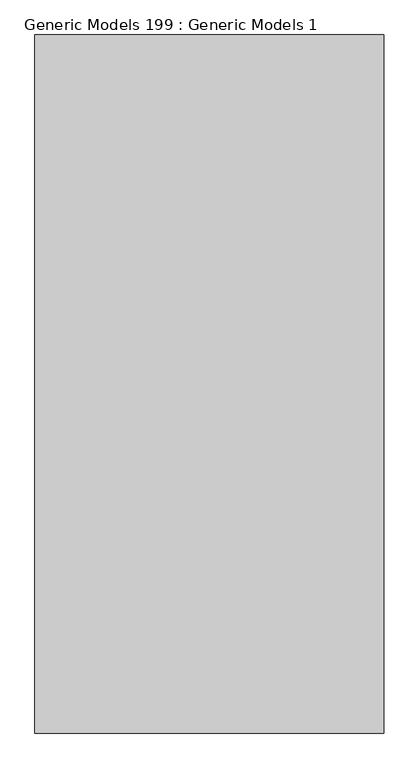
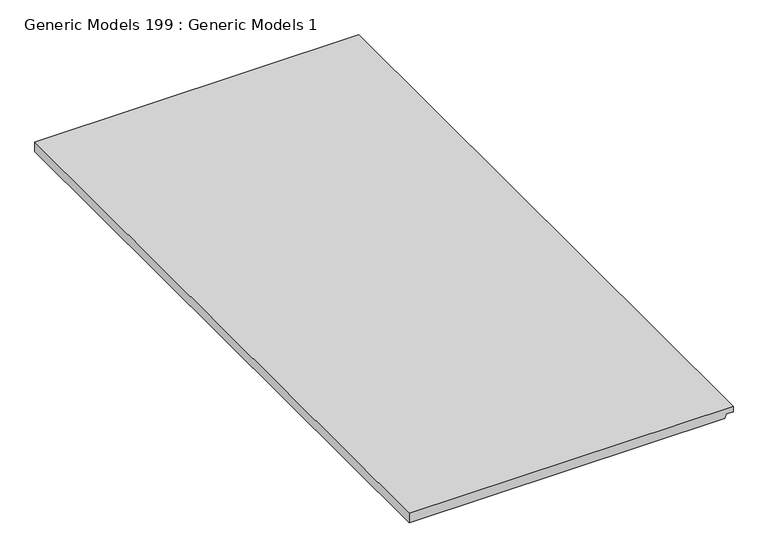
"""IFC4 building model written with IfcOpenShell, lengths in millimetres: proxy geometry, Generic Models 199 : Generic Models 1."""

import ifcopenshell
import ifcopenshell.guid

model = None  # the IFC model being written
_history = None  # IfcOwnerHistory: only IFC2X3 demands one
_inside = {}  # id of a spatial element -> (the spatial element, [elements in it])
_under = {}  # id of a project, library or spatial element -> (it, [spatial elements below it])
_declared = {}  # id of a project -> (the project, [libraries it declares])
_typed = {}  # id of a type object -> (the type object, [elements of that type])
_made_of = {}  # id of a material, layer set ... -> (it, [elements and type objects made of it])


def new_model(schema):
    """Start an empty IFC model of exactly this schema.

    Asked for "IFC4X3", IfcOpenShell would pick the latest addendum, in which some entities
    have other attributes; the version numbers below select the first issue.
    IFC2X3 requires an IfcOwnerHistory on every rooted entity: one is made here for all.
    """
    global model, _history
    if schema == "IFC4X3":
        model = ifcopenshell.file(schema_version=(4, 3, 0, 0))
    else:
        model = ifcopenshell.file(schema=schema)
    _inside.clear()
    _under.clear()
    _declared.clear()
    _typed.clear()
    _made_of.clear()
    _history = None
    if model.schema == "IFC2X3":
        org = make("IfcOrganization", Name="unknown")
        user = make(
            "IfcPersonAndOrganization",
            ThePerson=make("IfcPerson", FamilyName="unknown"),
            TheOrganization=org,
        )
        app = make(
            "IfcApplication",
            ApplicationDeveloper=org,
            Version="unknown",
            ApplicationFullName="unknown",
            ApplicationIdentifier="unknown",
        )
        _history = make(
            "IfcOwnerHistory",
            OwningUser=user,
            OwningApplication=app,
            ChangeAction="ADDED",
            CreationDate=0,
        )
    return model


def make(cls, **values):
    """One entity of the class cls with the attributes given. An attribute that is None is left unset."""
    return model.create_entity(
        cls, **{name: value for name, value in values.items() if value is not None}
    )


def rooted(cls, **values):
    """An entity with a GlobalId (a new one), such as an element, a storey or a relation."""
    return make(cls, GlobalId=ifcopenshell.guid.new(), OwnerHistory=_history, **values)


def si_unit(unit_type, name, prefix=None):
    """IfcSIUnit, for example si_unit("LENGTHUNIT", "METRE", prefix="MILLI")."""
    return make("IfcSIUnit", UnitType=unit_type, Prefix=prefix, Name=name)


def assignment(units):
    """IfcUnitAssignment: the units of a project."""
    return None if units is None else make("IfcUnitAssignment", Units=units)


def point(xyz):
    """IfcCartesianPoint."""
    return None if xyz is None else make("IfcCartesianPoint", Coordinates=xyz)


def direction(xyz):
    """IfcDirection."""
    return None if xyz is None else make("IfcDirection", DirectionRatios=xyz)


def frame(location, z_axis=None, x_axis=None):
    """IfcAxis2Placement3D, a coordinate frame: its origin and axes. An axis left out is left unset."""
    return make(
        "IfcAxis2Placement3D",
        Location=point(location),
        Axis=direction(z_axis),
        RefDirection=direction(x_axis),
    )


def origin():
    """The frame at (0, 0, 0) with its axes left unset."""
    return frame((0.0, 0.0, 0.0))


def place(relative_to, where):
    """IfcLocalPlacement: puts the frame where relative to a parent placement (None: the world)."""
    return make(
        "IfcLocalPlacement", PlacementRelTo=relative_to, RelativePlacement=where
    )


def context(
    kind, dimensions, precision=None, world=None, true_north=None, identifier=None
):
    """IfcGeometricRepresentationContext, for example the 3D "Model" context."""
    return make(
        "IfcGeometricRepresentationContext",
        ContextIdentifier=identifier,
        ContextType=kind,
        CoordinateSpaceDimension=dimensions,
        Precision=precision,
        WorldCoordinateSystem=world,
        TrueNorth=true_north,
    )


def project(units=None, contexts=None):
    """IfcProject with its units and contexts."""
    return rooted(
        "IfcProject",
        Name="project",
        RepresentationContexts=contexts,
        UnitsInContext=assignment(units),
    )


def spatial(cls, under=None, at=None, **own):
    """A site, building, storey or space (cls), placed at a placement, below another one or the project."""
    s = rooted(cls, ObjectPlacement=at, **own)
    if under is not None:
        _under.setdefault(under.id(), (under, []))[1].append(s)
    return s


def polyline(points):
    """IfcPolyline through the points."""
    return make("IfcPolyline", Points=[point(p) for p in points])


def outline(outer, holes=None, kind="AREA"):
    """IfcArbitraryClosedProfileDef: a profile drawn as a closed curve; with holes, ...WithVoids."""
    if holes is None:
        return make("IfcArbitraryClosedProfileDef", ProfileType=kind, OuterCurve=outer)
    return make(
        "IfcArbitraryProfileDefWithVoids",
        ProfileType=kind,
        OuterCurve=outer,
        InnerCurves=holes,
    )


def extrude(swept, where, along, depth):
    """IfcExtrudedAreaSolid: the profile swept, set in the frame where, extruded along a direction by depth."""
    return make(
        "IfcExtrudedAreaSolid",
        SweptArea=swept,
        Position=where,
        ExtrudedDirection=direction(along),
        Depth=depth,
    )


def shape(context_of_items, identifier, shape_type, items):
    """IfcShapeRepresentation: the items that make up one representation, for example the "Body"."""
    return make(
        "IfcShapeRepresentation",
        ContextOfItems=context_of_items,
        RepresentationIdentifier=identifier,
        RepresentationType=shape_type,
        Items=items,
    )


def source(mapping_origin, context_of_items, identifier, shape_type, items):
    """IfcRepresentationMap: a shape defined once, which mapped items show again and again."""
    return make(
        "IfcRepresentationMap",
        MappingOrigin=mapping_origin,
        MappedRepresentation=shape(context_of_items, identifier, shape_type, items),
    )


def transform(
    local_origin,
    x_axis=None,
    y_axis=None,
    z_axis=None,
    scale=None,
    scale2=None,
    scale3=None,
    uniform=True,
):
    """IfcCartesianTransformationOperator3D, or its non-uniform kind. x_axis, y_axis, z_axis: its Axis1, 2, 3."""
    if uniform:
        return make(
            "IfcCartesianTransformationOperator3D",
            Axis1=direction(x_axis),
            Axis2=direction(y_axis),
            LocalOrigin=point(local_origin),
            Scale=scale,
            Axis3=direction(z_axis),
        )
    return make(
        "IfcCartesianTransformationOperator3DnonUniform",
        Axis1=direction(x_axis),
        Axis2=direction(y_axis),
        LocalOrigin=point(local_origin),
        Scale=scale,
        Axis3=direction(z_axis),
        Scale2=scale2,
        Scale3=scale3,
    )


def mapped(mapping_source, mapping_target):
    """IfcMappedItem: shows the shape of a source again, moved by a transform."""
    return make(
        "IfcMappedItem", MappingSource=mapping_source, MappingTarget=mapping_target
    )


def made_of(thing, what):
    """Note that an element or type object is made of a material, layer set ...; save() writes the relation."""
    if what is not None:
        _made_of.setdefault(what.id(), (what, []))[1].append(thing)
    return thing


def element(
    cls,
    number,
    at=None,
    inside=None,
    cuts=None,
    type_object=None,
    material=None,
    context=None,
    identifier="Body",
    shape_type=None,
    held_by="IfcProductDefinitionShape",
    body=None,
    shapes=None,
    **own,
):
    """One element of the class cls, such as IfcWall. Its Tag is "e" and its number.

    at: its placement. inside: the storey or other place that contains it. cuts: it is an
    opening in that element (IfcRelVoidsElement). A single representation is given by context,
    identifier, shape_type and body (its items); several are given by shapes. held_by: the class
    of the entity that holds the representations. save() writes the other relations.
    """
    e = rooted(cls, Tag="e%d" % number, ObjectPlacement=at, **own)
    if body is not None:
        shapes = [shape(context, identifier, shape_type, body)]
    if shapes is not None:
        e.Representation = make(held_by, Representations=shapes)
    if inside is not None:
        _inside.setdefault(inside.id(), (inside, []))[1].append(e)
    if cuts is not None:
        rooted(
            "IfcRelVoidsElement", RelatingBuildingElement=cuts, RelatedOpeningElement=e
        )
    if type_object is not None:
        _typed.setdefault(type_object.id(), (type_object, []))[1].append(e)
    return made_of(e, material)


def aggregate(whole, parts):
    """IfcRelAggregates: a whole, such as a stair, and the parts it consists of."""
    return rooted("IfcRelAggregates", RelatingObject=whole, RelatedObjects=parts)


def save(model, path):
    """Write the relations noted so far, then the file.

    IfcRelAggregates (storeys below a building ...), IfcRelContainedInSpatialStructure (elements
    in a storey), IfcRelDefinesByType, IfcRelAssociatesMaterial and IfcRelDeclares: one each for
    every whole, place, type object, material and project.
    """
    for whole, parts in _under.values():
        aggregate(whole, parts)
    for where, things in _inside.values():
        rooted(
            "IfcRelContainedInSpatialStructure",
            RelatedElements=things,
            RelatingStructure=where,
        )
    for kind, things in _typed.values():
        rooted("IfcRelDefinesByType", RelatedObjects=things, RelatingType=kind)
    for what, things in _made_of.values():
        rooted("IfcRelAssociatesMaterial", RelatedObjects=things, RelatingMaterial=what)
    for by, libraries in _declared.values():
        rooted("IfcRelDeclares", RelatingContext=by, RelatedDefinitions=libraries)
    model.write(path)


def generic_models_199_generic_models_1_28f40251(model_context):
    return source(origin(), model_context, "Body", "SweptSolid", [
        extrude(outline(polyline([(2253.330428, 49662.5798593), (2253.330428, 49052.9798593), (2234.280428, 49052.9798593), (2234.280428, 49646.9908455), (2242.217928, 49649.8798593), (2242.217928, 49662.5798593), (2253.330428, 49662.5798593)])), frame((0.0, 0.0, 0.0), z_axis=(0.0, 1.0, 0.0), x_axis=(0.0, 0.0, 1.0)), (0.0, 0.0, 1.0), 1219.2),
    ])


if __name__ == "__main__":
    model = new_model("IFC4")
    model_context = context("Model", 3, world=origin())
    ifc_project = project(units=[si_unit("LENGTHUNIT", "METRE", prefix="MILLI")], contexts=[model_context])
    site = spatial("IfcSite", under=ifc_project)
    building = spatial("IfcBuilding", under=site)
    placement = place(None, origin())
    generic_models_199_generic_models_1_shape = generic_models_199_generic_models_1_28f40251(model_context)
    element("IfcBuildingElementProxy", 1, Name="Generic Models 199 : Generic Models 1", ObjectType="Generic Models 199 : Generic Models 1", at=placement, inside=building, context=model_context, shape_type="MappedRepresentation", body=[
        mapped(generic_models_199_generic_models_1_shape, transform((0.0, 0.0, 0.0), x_axis=(1.0, 0.0, 0.0), y_axis=(0.0, 1.0, 0.0), z_axis=(0.0, 0.0, 1.0))),
    ])
    save(model, "model.ifc")

# Revit data of these elements
# Element 1 (IfcBuildingElementProxy, "Generic Models 199 : Generic Models 1")
#   Materials on its faces: "CEILING AS SCHEDULED"
# Materials
#   "CEILING AS SCHEDULED": class "Generic", colour RGB 255 255 255, transparency 0, Cost = 0
